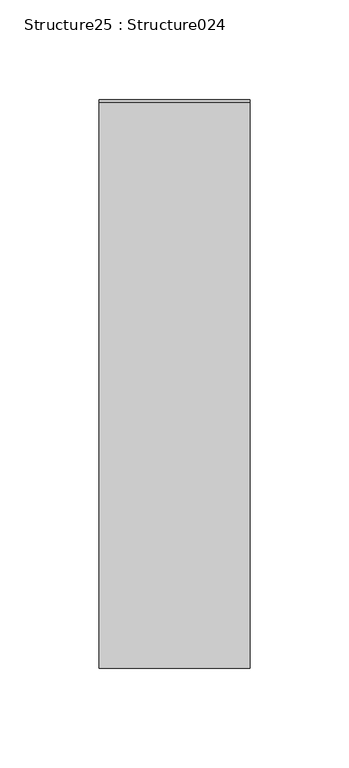
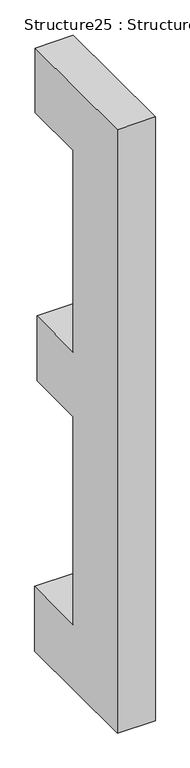
"""IFC4 building model written with IfcOpenShell, lengths in millimetres: proxy geometry, Structure25 : Structure024."""

from ifc_helpers import new_model, si_unit, frame, origin, place, context, project, spatial, polyline, outline, extrude, source, transform, mapped, element, save


def structure25_structure024_8bdedd8d(model_context):
    return source(origin(), model_context, "Body", "SweptSolid", [
        extrude(outline(polyline([(1280.4310236, 0.0), (1280.4310236, -285.3583213), (1143.2462515, -285.3583213), (1143.2462515, -153.6692086), (715.2083459, -153.6692086), (715.2083459, -279.8635091), (578.024421, -279.8635091), (578.024421, -153.6692086), (137.1830777, -153.6692086), (137.1830777, -287.1823008), (0.0, -287.1823008), (0.0, 0.0), (1280.4310236, 0.0)])), frame((-35624.0862846, 278189.4791919, 4479.6663888), z_axis=(1.0, 0.0, 1.354250045437766e-12), x_axis=(-1.354250045437766e-12, 0.0, 1.0)), (0.0, 0.0, 1.0), 76.2),
    ])


if __name__ == "__main__":
    model = new_model("IFC4")
    model_context = context("Model", 3, world=origin())
    ifc_project = project(units=[si_unit("LENGTHUNIT", "METRE", prefix="MILLI")], contexts=[model_context])
    site = spatial("IfcSite", under=ifc_project)
    building = spatial("IfcBuilding", under=site)
    placement = place(None, origin())
    structure25_structure024_shape = structure25_structure024_8bdedd8d(model_context)
    element("IfcBuildingElementProxy", 1, Name="Structure25 : Structure024", ObjectType="Structure25 : Structure024", at=placement, inside=building, context=model_context, shape_type="MappedRepresentation", body=[
        mapped(structure25_structure024_shape, transform((0.0, 0.0, 0.0), x_axis=(1.0, 0.0, 0.0), y_axis=(0.0, 1.0, 0.0), z_axis=(0.0, 0.0, 1.0))),
    ])
    save(model, "model.ifc")

# Revit data of these elements
# Type "Structure25 : Structure024"
#   NameOverride = "Structure024"
# Element 1 (IfcBuildingElementProxy, "Structure25 : Structure024")
#   Materials on its faces: "BRUSHED ALUMINUM LETTERING"
# Materials
#   "BRUSHED ALUMINUM LETTERING": class "Unassigned", colour RGB 169 181 186, transparency 0, Cost = 0
